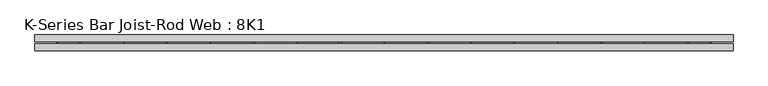
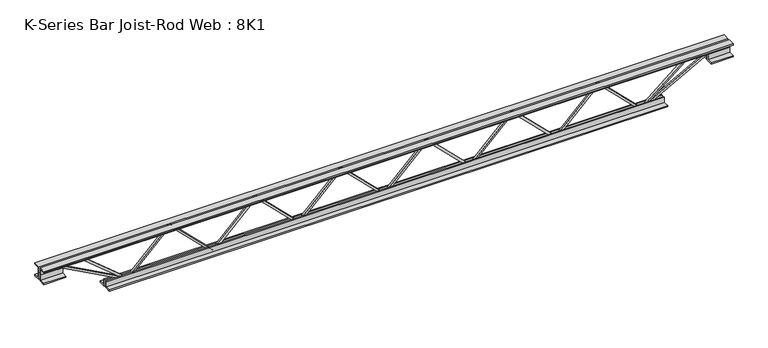
"""IFC4 building model written with IfcOpenShell, lengths in millimetres: beam geometry, K-Series Bar Joist-Rod Web : 8K1."""

from ifc_helpers import new_model, si_unit, frame, origin, place, context, project, spatial, polyline, outline, extrude, source, transform, mapped, element, save


def k_series_bar_joist_rod_web_8k1_a298f018(model_context):
    return source(origin(), model_context, "Body", "SweptSolid", [
        extrude(outline(polyline([(-90.4875, 398.8522061), (-100.0125, 398.8522061), (-100.0125, 403.981188), (90.4875, 597.057291), (90.4875, 599.4993272), (-100.0125, 792.5754302), (-100.0125, 797.7044121), (-90.4875, 797.7044121), (-90.4875, 796.483394), (100.0125, 603.407291), (100.0125, 593.1493272), (-90.4875, 400.0732241), (-90.4875, 398.8522061)])), frame((0.0, -4.7625, 0.0), z_axis=(0.0, 1.0, 0.0), x_axis=(0.0, 0.0, 1.0)), (0.0, 0.0, 1.0), 9.525),
        extrude(outline(polyline([(-90.4875, 0.0), (-100.0125, 0.0), (-100.0125, 5.1289819), (90.4875, 198.205085), (90.4875, 200.6471211), (-100.0125, 393.7232241), (-100.0125, 398.8522061), (-90.4875, 398.8522061), (-90.4875, 397.631188), (100.0125, 204.555085), (100.0125, 194.2971211), (-90.4875, 1.2210181), (-90.4875, 0.0)])), frame((0.0, -4.7625, 0.0), z_axis=(0.0, 1.0, 0.0), x_axis=(0.0, 0.0, 1.0)), (0.0, 0.0, 1.0), 9.525),
        extrude(outline(polyline([(-90.4875, -398.8522061), (-100.0125, -398.8522061), (-100.0125, -393.7232241), (90.4875, -200.6471211), (90.4875, -198.205085), (-100.0125, -5.1289819), (-100.0125, 0.0), (-90.4875, 0.0), (-90.4875, -1.2210181), (100.0125, -194.2971211), (100.0125, -204.555085), (-90.4875, -397.631188), (-90.4875, -398.8522061)])), frame((0.0, -4.7625, 0.0), z_axis=(0.0, 1.0, 0.0), x_axis=(0.0, 0.0, 1.0)), (0.0, 0.0, 1.0), 9.525),
        extrude(outline(polyline([(-90.4875, -797.7044121), (-100.0125, -797.7044121), (-100.0125, -792.5754302), (90.4875, -599.4993272), (90.4875, -597.057291), (-100.0125, -403.981188), (-100.0125, -398.8522061), (-90.4875, -398.8522061), (-90.4875, -400.0732241), (100.0125, -593.1493272), (100.0125, -603.407291), (-90.4875, -796.483394), (-90.4875, -797.7044121)])), frame((0.0, -4.7625, 0.0), z_axis=(0.0, 1.0, 0.0), x_axis=(0.0, 0.0, 1.0)), (0.0, 0.0, 1.0), 9.525),
        extrude(outline(polyline([(-90.4875, 797.7044121), (-100.0125, 797.7044121), (-100.0125, 802.833394), (90.4875, 995.9094971), (90.4875, 998.3515332), (-100.0125, 1191.4276362), (-100.0125, 1196.5566182), (-90.4875, 1196.5566182), (-90.4875, 1195.3356001), (100.0125, 1002.2594971), (100.0125, 992.0015332), (-90.4875, 798.9254302), (-90.4875, 797.7044121)])), frame((0.0, -4.7625, 0.0), z_axis=(0.0, 1.0, 0.0), x_axis=(0.0, 0.0, 1.0)), (0.0, 0.0, 1.0), 9.525),
        extrude(outline(polyline([(-90.4875, -1196.5566182), (-100.0125, -1196.5566182), (-100.0125, -1191.4276362), (90.4875, -998.3515332), (90.4875, -995.9094971), (-100.0125, -802.833394), (-100.0125, -797.7044121), (-90.4875, -797.7044121), (-90.4875, -798.9254302), (100.0125, -992.0015332), (100.0125, -1002.2594971), (-90.4875, -1195.3356001), (-90.4875, -1196.5566182)])), frame((0.0, -4.7625, 0.0), z_axis=(0.0, 1.0, 0.0), x_axis=(0.0, 0.0, 1.0)), (0.0, 0.0, 1.0), 9.525),
        extrude(outline(polyline([(4.7625, 101.6), (36.5125, 101.6), (36.5125, 95.25), (11.1125, 95.25), (11.1125, 69.85), (4.7625, 69.85), (4.7625, 101.6)])), frame((-1602.9566182, 0.0, 0.0), z_axis=(1.0, 0.0, 0.0), x_axis=(0.0, 1.0, 0.0)), (0.0, 0.0, 1.0), 3205.9132363),
        extrude(outline(polyline([(-4.7625, 101.6), (-4.7625, 69.85), (-11.1125, 69.85), (-11.1125, 95.25), (-36.5125, 95.25), (-36.5125, 101.6), (-4.7625, 101.6)])), frame((-1602.9566182, 0.0, 0.0), z_axis=(1.0, 0.0, 0.0), x_axis=(0.0, 1.0, 0.0)), (0.0, 0.0, 1.0), 3205.9132363),
        extrude(outline(polyline([(-4.7625, 38.1), (-36.5125, 38.1), (-36.5125, 44.45), (-11.1125, 44.45), (-11.1125, 69.85), (-4.7625, 69.85), (-4.7625, 38.1)])), frame((-1602.9566182, 0.0, 0.0), z_axis=(1.0, 0.0, 0.0), x_axis=(0.0, 1.0, 0.0)), (0.0, 0.0, 1.0), 101.6),
        extrude(outline(polyline([(36.5125, 38.1), (4.7625, 38.1), (4.7625, 69.85), (11.1125, 69.85), (11.1125, 44.45), (36.5125, 44.45), (36.5125, 38.1)])), frame((-1602.9566182, 0.0, 0.0), z_axis=(1.0, 0.0, 0.0), x_axis=(0.0, 1.0, 0.0)), (0.0, 0.0, 1.0), 101.6),
        extrude(outline(polyline([(4.7625, 38.1), (4.7625, 69.85), (11.1125, 69.85), (11.1125, 44.45), (36.5125, 44.45), (36.5125, 38.1), (4.7625, 38.1)])), frame((1501.3566182, 0.0, 0.0), z_axis=(1.0, 0.0, 0.0), x_axis=(0.0, 1.0, 0.0)), (0.0, 0.0, 1.0), 101.6),
        extrude(outline(polyline([(-4.7625, 38.1), (-36.5125, 38.1), (-36.5125, 44.45), (-11.1125, 44.45), (-11.1125, 69.85), (-4.7625, 69.85), (-4.7625, 38.1)])), frame((1501.3566182, 0.0, 0.0), z_axis=(1.0, 0.0, 0.0), x_axis=(0.0, 1.0, 0.0)), (0.0, 0.0, 1.0), 101.6),
        extrude(outline(polyline([(4.7625, -101.6), (4.7625, -69.85), (11.1125, -69.85), (11.1125, -95.25), (36.5125, -95.25), (36.5125, -101.6), (4.7625, -101.6)])), frame((-1298.1566182, 0.0, 0.0), z_axis=(1.0, 0.0, 0.0), x_axis=(0.0, 1.0, 0.0)), (0.0, 0.0, 1.0), 2596.3132363),
        extrude(outline(polyline([(-4.7625, -101.6), (-36.5125, -101.6), (-36.5125, -95.25), (-11.1125, -95.25), (-11.1125, -69.85), (-4.7625, -69.85), (-4.7625, -101.6)])), frame((-1298.1566182, 0.0, 0.0), z_axis=(1.0, 0.0, 0.0), x_axis=(0.0, 1.0, 0.0)), (0.0, 0.0, 1.0), 2596.3132363),
        extrude(outline(polyline([(0.0, -9.525), (0.0, 0.0), (346.6425392, 0.0), (346.6425392, -9.525), (0.0, -9.525)])), frame((-1503.6249167, 4.7625, 65.662372), z_axis=(0.4762831485400797, 0.0, 0.8792919665371386), x_axis=(0.8792919665371386, 0.0, -0.4762831485400797)), (0.0, 0.0, 1.0), 9.525),
        extrude(outline(polyline([(0.0, -9.525), (0.0, 0.0), (258.8991706, 0.0), (258.8991706, -9.525), (0.0, -9.525)])), frame((-1399.0197674, 4.7625, 66.1815185), z_axis=(0.6376999956317555, 0.0, 0.7702848275613763), x_axis=(0.7702848275613763, 0.0, -0.6376999956317555)), (0.0, 0.0, 1.0), 9.525),
        extrude(outline(polyline([(0.0, -9.525), (0.0, 0.0), (346.6425392, 0.0), (346.6425392, -9.525), (0.0, -9.525)])), frame((1503.6249167, -4.7625, 65.662372), z_axis=(-0.47628314854004167, 0.0, 0.8792919665371591), x_axis=(-0.8792919665371591, 0.0, -0.47628314854004167)), (0.0, 0.0, 1.0), 9.525),
        extrude(outline(polyline([(0.0, -9.525), (0.0, 0.0), (258.8991706, 0.0), (258.8991706, -9.525), (0.0, -9.525)])), frame((1399.0197674, -4.7625, 66.1815185), z_axis=(-0.6376999956317273, 0.0, 0.7702848275613995), x_axis=(-0.7702848275613995, 0.0, -0.6376999956317273)), (0.0, 0.0, 1.0), 9.525),
    ])


if __name__ == "__main__":
    model = new_model("IFC4")
    model_context = context("Model", 3, world=origin())
    ifc_project = project(units=[si_unit("LENGTHUNIT", "METRE", prefix="MILLI")], contexts=[model_context])
    site = spatial("IfcSite", under=ifc_project)
    building = spatial("IfcBuilding", under=site)
    placement = place(None, origin())
    k_series_bar_joist_rod_web_8k1_shape = k_series_bar_joist_rod_web_8k1_a298f018(model_context)
    element("IfcBeam", 1, ObjectType="K-Series Bar Joist-Rod Web : 8K1", at=placement, inside=building, context=model_context, shape_type="MappedRepresentation", body=[
        mapped(k_series_bar_joist_rod_web_8k1_shape, transform((0.0, 0.0, 0.0), x_axis=(1.0, 0.0, 0.0), y_axis=(0.0, 1.0, 0.0), z_axis=(0.0, 0.0, 1.0))),
    ])
    save(model, "model.ifc")

# Revit data of these elements
# Type "K-Series Bar Joist-Rod Web : 8K1"
#   Assembly Code = "B1010350"
#   Wt = 5.1
#   Web Thickness = 0' - 0 3/8"
#   Start Offset [instance default] = 0' - 0"
#   Start Extension [instance default] = 0' - 0"
#   Seat Length = 0' - 4"
#   Seat Depth = 0' - 2 1/2"
#   PanelArrayLength [instance default] = 21' - 4"
#   Panel [instance default] = 1' - 4"
#   End Offset [instance default] = 0' - 0"
#   End Extension [instance default] = 0' - 0"
#   End Panel = 1' - 4"
#   Cord Leg = 0' - 1 1/4"
#   Chord Thickness = 0' - 0 1/4"
#   Length [instance default] = 24' - 0"
#   Depth = 0' - 8"
#   PanelArrayNum [instance default] = 16
#   Rendering Material = none
# Element 1 (IfcBeam, "K-Series Bar Joist-Rod Web : 8K1")
#   PanelArrayLength = 7' - 10.21706"
#   Panel = 1' - 3.70284"
#   PanelArrayNum = 6
